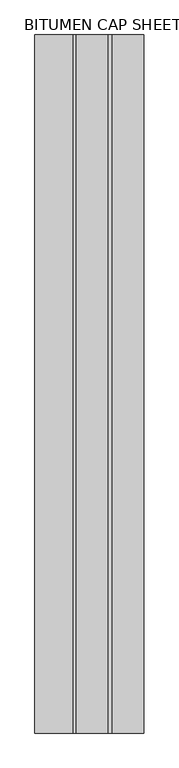
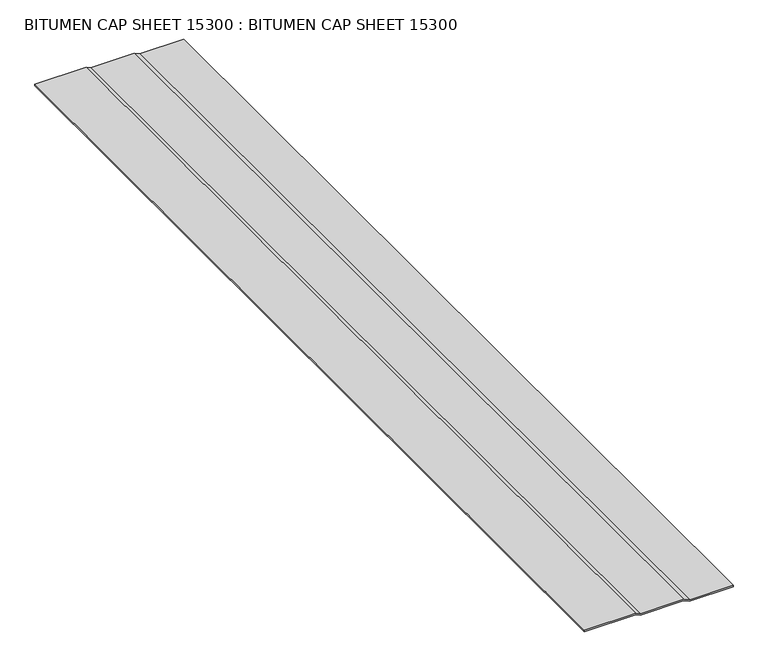
"""IFC4 building model written with IfcOpenShell, lengths in millimetres: proxy geometry, BITUMEN CAP SHEET 15300 : BITUMEN CAP SHEET 15300."""

import ifcopenshell
import ifcopenshell.guid

model = None  # the IFC model being written
_history = None  # IfcOwnerHistory: only IFC2X3 demands one
_inside = {}  # id of a spatial element -> (the spatial element, [elements in it])
_under = {}  # id of a project, library or spatial element -> (it, [spatial elements below it])
_declared = {}  # id of a project -> (the project, [libraries it declares])
_typed = {}  # id of a type object -> (the type object, [elements of that type])
_made_of = {}  # id of a material, layer set ... -> (it, [elements and type objects made of it])


def new_model(schema):
    """Start an empty IFC model of exactly this schema.

    Asked for "IFC4X3", IfcOpenShell would pick the latest addendum, in which some entities
    have other attributes; the version numbers below select the first issue.
    IFC2X3 requires an IfcOwnerHistory on every rooted entity: one is made here for all.
    """
    global model, _history
    if schema == "IFC4X3":
        model = ifcopenshell.file(schema_version=(4, 3, 0, 0))
    else:
        model = ifcopenshell.file(schema=schema)
    _inside.clear()
    _under.clear()
    _declared.clear()
    _typed.clear()
    _made_of.clear()
    _history = None
    if model.schema == "IFC2X3":
        org = make("IfcOrganization", Name="unknown")
        user = make(
            "IfcPersonAndOrganization",
            ThePerson=make("IfcPerson", FamilyName="unknown"),
            TheOrganization=org,
        )
        app = make(
            "IfcApplication",
            ApplicationDeveloper=org,
            Version="unknown",
            ApplicationFullName="unknown",
            ApplicationIdentifier="unknown",
        )
        _history = make(
            "IfcOwnerHistory",
            OwningUser=user,
            OwningApplication=app,
            ChangeAction="ADDED",
            CreationDate=0,
        )
    return model


def make(cls, **values):
    """One entity of the class cls with the attributes given. An attribute that is None is left unset."""
    return model.create_entity(
        cls, **{name: value for name, value in values.items() if value is not None}
    )


def rooted(cls, **values):
    """An entity with a GlobalId (a new one), such as an element, a storey or a relation."""
    return make(cls, GlobalId=ifcopenshell.guid.new(), OwnerHistory=_history, **values)


def si_unit(unit_type, name, prefix=None):
    """IfcSIUnit, for example si_unit("LENGTHUNIT", "METRE", prefix="MILLI")."""
    return make("IfcSIUnit", UnitType=unit_type, Prefix=prefix, Name=name)


def assignment(units):
    """IfcUnitAssignment: the units of a project."""
    return None if units is None else make("IfcUnitAssignment", Units=units)


def point(xyz):
    """IfcCartesianPoint."""
    return None if xyz is None else make("IfcCartesianPoint", Coordinates=xyz)


def direction(xyz):
    """IfcDirection."""
    return None if xyz is None else make("IfcDirection", DirectionRatios=xyz)


def frame(location, z_axis=None, x_axis=None):
    """IfcAxis2Placement3D, a coordinate frame: its origin and axes. An axis left out is left unset."""
    return make(
        "IfcAxis2Placement3D",
        Location=point(location),
        Axis=direction(z_axis),
        RefDirection=direction(x_axis),
    )


def origin():
    """The frame at (0, 0, 0) with its axes left unset."""
    return frame((0.0, 0.0, 0.0))


def place(relative_to, where):
    """IfcLocalPlacement: puts the frame where relative to a parent placement (None: the world)."""
    return make(
        "IfcLocalPlacement", PlacementRelTo=relative_to, RelativePlacement=where
    )


def context(
    kind, dimensions, precision=None, world=None, true_north=None, identifier=None
):
    """IfcGeometricRepresentationContext, for example the 3D "Model" context."""
    return make(
        "IfcGeometricRepresentationContext",
        ContextIdentifier=identifier,
        ContextType=kind,
        CoordinateSpaceDimension=dimensions,
        Precision=precision,
        WorldCoordinateSystem=world,
        TrueNorth=true_north,
    )


def project(units=None, contexts=None):
    """IfcProject with its units and contexts."""
    return rooted(
        "IfcProject",
        Name="project",
        RepresentationContexts=contexts,
        UnitsInContext=assignment(units),
    )


def spatial(cls, under=None, at=None, **own):
    """A site, building, storey or space (cls), placed at a placement, below another one or the project."""
    s = rooted(cls, ObjectPlacement=at, **own)
    if under is not None:
        _under.setdefault(under.id(), (under, []))[1].append(s)
    return s


def polyline(points):
    """IfcPolyline through the points."""
    return make("IfcPolyline", Points=[point(p) for p in points])


def outline(outer, holes=None, kind="AREA"):
    """IfcArbitraryClosedProfileDef: a profile drawn as a closed curve; with holes, ...WithVoids."""
    if holes is None:
        return make("IfcArbitraryClosedProfileDef", ProfileType=kind, OuterCurve=outer)
    return make(
        "IfcArbitraryProfileDefWithVoids",
        ProfileType=kind,
        OuterCurve=outer,
        InnerCurves=holes,
    )


def extrude(swept, where, along, depth):
    """IfcExtrudedAreaSolid: the profile swept, set in the frame where, extruded along a direction by depth."""
    return make(
        "IfcExtrudedAreaSolid",
        SweptArea=swept,
        Position=where,
        ExtrudedDirection=direction(along),
        Depth=depth,
    )


def shape(context_of_items, identifier, shape_type, items):
    """IfcShapeRepresentation: the items that make up one representation, for example the "Body"."""
    return make(
        "IfcShapeRepresentation",
        ContextOfItems=context_of_items,
        RepresentationIdentifier=identifier,
        RepresentationType=shape_type,
        Items=items,
    )


def source(mapping_origin, context_of_items, identifier, shape_type, items):
    """IfcRepresentationMap: a shape defined once, which mapped items show again and again."""
    return make(
        "IfcRepresentationMap",
        MappingOrigin=mapping_origin,
        MappedRepresentation=shape(context_of_items, identifier, shape_type, items),
    )


def transform(
    local_origin,
    x_axis=None,
    y_axis=None,
    z_axis=None,
    scale=None,
    scale2=None,
    scale3=None,
    uniform=True,
):
    """IfcCartesianTransformationOperator3D, or its non-uniform kind. x_axis, y_axis, z_axis: its Axis1, 2, 3."""
    if uniform:
        return make(
            "IfcCartesianTransformationOperator3D",
            Axis1=direction(x_axis),
            Axis2=direction(y_axis),
            LocalOrigin=point(local_origin),
            Scale=scale,
            Axis3=direction(z_axis),
        )
    return make(
        "IfcCartesianTransformationOperator3DnonUniform",
        Axis1=direction(x_axis),
        Axis2=direction(y_axis),
        LocalOrigin=point(local_origin),
        Scale=scale,
        Axis3=direction(z_axis),
        Scale2=scale2,
        Scale3=scale3,
    )


def mapped(mapping_source, mapping_target):
    """IfcMappedItem: shows the shape of a source again, moved by a transform."""
    return make(
        "IfcMappedItem", MappingSource=mapping_source, MappingTarget=mapping_target
    )


def made_of(thing, what):
    """Note that an element or type object is made of a material, layer set ...; save() writes the relation."""
    if what is not None:
        _made_of.setdefault(what.id(), (what, []))[1].append(thing)
    return thing


def element(
    cls,
    number,
    at=None,
    inside=None,
    cuts=None,
    type_object=None,
    material=None,
    context=None,
    identifier="Body",
    shape_type=None,
    held_by="IfcProductDefinitionShape",
    body=None,
    shapes=None,
    **own,
):
    """One element of the class cls, such as IfcWall. Its Tag is "e" and its number.

    at: its placement. inside: the storey or other place that contains it. cuts: it is an
    opening in that element (IfcRelVoidsElement). A single representation is given by context,
    identifier, shape_type and body (its items); several are given by shapes. held_by: the class
    of the entity that holds the representations. save() writes the other relations.
    """
    e = rooted(cls, Tag="e%d" % number, ObjectPlacement=at, **own)
    if body is not None:
        shapes = [shape(context, identifier, shape_type, body)]
    if shapes is not None:
        e.Representation = make(held_by, Representations=shapes)
    if inside is not None:
        _inside.setdefault(inside.id(), (inside, []))[1].append(e)
    if cuts is not None:
        rooted(
            "IfcRelVoidsElement", RelatingBuildingElement=cuts, RelatedOpeningElement=e
        )
    if type_object is not None:
        _typed.setdefault(type_object.id(), (type_object, []))[1].append(e)
    return made_of(e, material)


def aggregate(whole, parts):
    """IfcRelAggregates: a whole, such as a stair, and the parts it consists of."""
    return rooted("IfcRelAggregates", RelatingObject=whole, RelatedObjects=parts)


def save(model, path):
    """Write the relations noted so far, then the file.

    IfcRelAggregates (storeys below a building ...), IfcRelContainedInSpatialStructure (elements
    in a storey), IfcRelDefinesByType, IfcRelAssociatesMaterial and IfcRelDeclares: one each for
    every whole, place, type object, material and project.
    """
    for whole, parts in _under.values():
        aggregate(whole, parts)
    for where, things in _inside.values():
        rooted(
            "IfcRelContainedInSpatialStructure",
            RelatedElements=things,
            RelatingStructure=where,
        )
    for kind, things in _typed.values():
        rooted("IfcRelDefinesByType", RelatedObjects=things, RelatingType=kind)
    for what, things in _made_of.values():
        rooted("IfcRelAssociatesMaterial", RelatedObjects=things, RelatingMaterial=what)
    for by, libraries in _declared.values():
        rooted("IfcRelDeclares", RelatingContext=by, RelatedDefinitions=libraries)
    model.write(path)


def bitumen_cap_sheet_15300_bitumen_cap_sheet_15300_313e2dc3(model_context):
    return source(origin(), model_context, "Body", "SweptSolid", [
        extrude(outline(polyline([(40259.2002678, -2469.2761954), (40262.3752678, -2469.2761954), (40262.3752678, -2560.795457), (40267.6612773, -2573.2602756), (40267.6612773, -2663.9440313), (40271.9940719, -2673.6609328), (40271.9940719, -2781.5474293), (40268.8188423, -2781.5474293), (40268.8188423, -2674.3362183), (40264.4862773, -2664.6198318), (40264.4862773, -2573.9056756), (40259.2002678, -2561.440857), (40259.2002678, -2469.2761954)])), frame((0.0, -1052.8906574, 0.0), z_axis=(0.0, 1.0, 0.0), x_axis=(0.0, 0.0, 1.0)), (0.0, 0.0, 1.0), 2000.25),
    ])


if __name__ == "__main__":
    model = new_model("IFC4")
    model_context = context("Model", 3, world=origin())
    ifc_project = project(units=[si_unit("LENGTHUNIT", "METRE", prefix="MILLI")], contexts=[model_context])
    site = spatial("IfcSite", under=ifc_project)
    building = spatial("IfcBuilding", under=site)
    placement = place(None, origin())
    bitumen_cap_sheet_15300_bitumen_cap_sheet_15300_shape = bitumen_cap_sheet_15300_bitumen_cap_sheet_15300_313e2dc3(model_context)
    element("IfcBuildingElementProxy", 1, Name="BITUMEN CAP SHEET 15300 : BITUMEN CAP SHEET 15300", ObjectType="BITUMEN CAP SHEET 15300 : BITUMEN CAP SHEET 15300", at=placement, inside=building, context=model_context, shape_type="MappedRepresentation", body=[
        mapped(bitumen_cap_sheet_15300_bitumen_cap_sheet_15300_shape, transform((0.0, 0.0, 0.0), x_axis=(1.0, 0.0, 0.0), y_axis=(0.0, 1.0, 0.0), z_axis=(0.0, 0.0, 1.0))),
    ])
    save(model, "model.ifc")

# Revit data of these elements
# Type "BITUMEN CAP SHEET 15300 : BITUMEN CAP SHEET 15300"
#   NameOverride = "BITUMEN CAP SHEET"
# Element 1 (IfcBuildingElementProxy, "BITUMEN CAP SHEET 15300 : BITUMEN CAP SHEET 15300")
#   Materials on its faces: "MODIFIED BITUMEN GRANULE SURFACED CAP SHEET"
# Materials
#   "MODIFIED BITUMEN GRANULE SURFACED CAP SHEET": class "Unassigned", colour RGB 85 85 127, transparency 0
